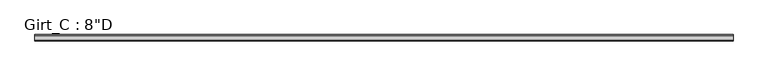
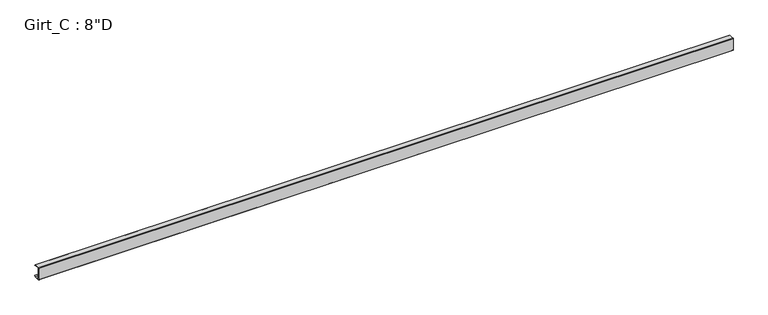
"""IFC4 building model written with IfcOpenShell, lengths in millimetres: beam geometry."""

from ifc_helpers import new_model, si_unit, point, frame, frame_2d, origin, place, context, project, spatial, polyline, circle_curve, trimmed, segment, composite_curve, outline, extrude, source, transform, mapped, element, save


def beam_73cb32fd(model_context):
    return source(origin(), model_context, "Body", "SweptSolid", [
        extrude(outline(composite_curve([segment(polyline([(87.5109375, 101.6), (99.7560415, 87.0068534), (97.6278742, 85.221109), (86.2154765, 98.821875), (3.3005807, 98.821875)]), True, "CONTINUOUS"), segment(trimmed(circle_curve(frame_2d((3.3741066, 96.8381931)), 1.9850441), [point((3.3005807, 98.821875))], [point((1.3890625, 96.8381931))], True, "CARTESIAN"), True, "CONTINUOUS"), segment(polyline([(1.3890625, 96.8381931), (1.3890625, -96.8389339)]), True, "CONTINUOUS"), segment(trimmed(circle_curve(frame_2d((3.3748024, -96.8389339)), 1.9857399), [point((1.3890625, -96.8389339))], [point((3.2694106, -98.821875))], True, "CARTESIAN"), True, "CONTINUOUS"), segment(polyline([(3.2694106, -98.821875), (86.2154765, -98.821875), (97.6510975, -85.1934327), (99.7792647, -86.979177), (87.5109375, -101.6), (3.3734375, -101.6)]), True, "CONTINUOUS"), segment(trimmed(circle_curve(frame_2d((3.3734375, -96.8375)), 4.7625), [point((3.3734375, -101.6))], [point((-1.3890625, -96.8375))], False, "CARTESIAN"), True, "CONTINUOUS"), segment(polyline([(-1.3890625, -96.8375), (-1.3890625, 96.8375)]), True, "CONTINUOUS"), segment(trimmed(circle_curve(frame_2d((3.3734375, 96.8375)), 4.7625), [point((-1.3890625, 96.8375))], [point((3.3734375, 101.6))], False, "CARTESIAN"), True, "CONTINUOUS"), segment(polyline([(3.3734375, 101.6), (87.5109375, 101.6)]), True, "CONTINUOUS")], self_intersect=False)), frame((-5643.4399169, 0.0, 0.0), z_axis=(1.0, 0.0, 0.0), x_axis=(0.0, 1.0, 0.0)), (0.0, 0.0, 1.0), 11286.8798339),
    ])


if __name__ == "__main__":
    model = new_model("IFC4")
    model_context = context("Model", 3, world=origin())
    ifc_project = project(units=[si_unit("LENGTHUNIT", "METRE", prefix="MILLI")], contexts=[model_context])
    site = spatial("IfcSite", under=ifc_project)
    building = spatial("IfcBuilding", under=site)
    placement = place(None, origin())
    beam_shape = beam_73cb32fd(model_context)
    element("IfcBeam", 1, ObjectType="Girt_C : 8\"D", at=placement, inside=building, context=model_context, shape_type="MappedRepresentation", body=[
        mapped(beam_shape, transform((0.0, 0.0, 0.0), x_axis=(1.0, 0.0, 0.0), y_axis=(0.0, 1.0, 0.0), z_axis=(0.0, 0.0, 1.0))),
    ])
    save(model, "model.ifc")

# Revit data of these elements
# Type "Girt_C : 8\"D"
#   half leg = 0' - 1 3/4"
#   Web_Thickness = 0' - 0 7/64"
#   Length [instance default] = 10' - 0"
#   Leg_1 = 0' - 3 1/2"
#   Height = 0' - 8"
#   Structural Material [instance default] = none
# Element 1 (IfcBeam, "Girt_C : 8\"D")
#   Structural Material = GALVANIZED 'CEE' SECTION (8.0x3.5C - SEE STRUCT. DWGS)
#   Materials on its faces: "GALVANIZED 'CEE' SECTION (8.0x3.5C - SEE STRUCT. DWGS)"
# Materials
#   "GALVANIZED 'CEE' SECTION (8.0x3.5C - SEE STRUCT. DWGS)": class "Metal", colour RGB 137 146 153, transparency 0, Description = "Steel, mill finish", Cost = 0
